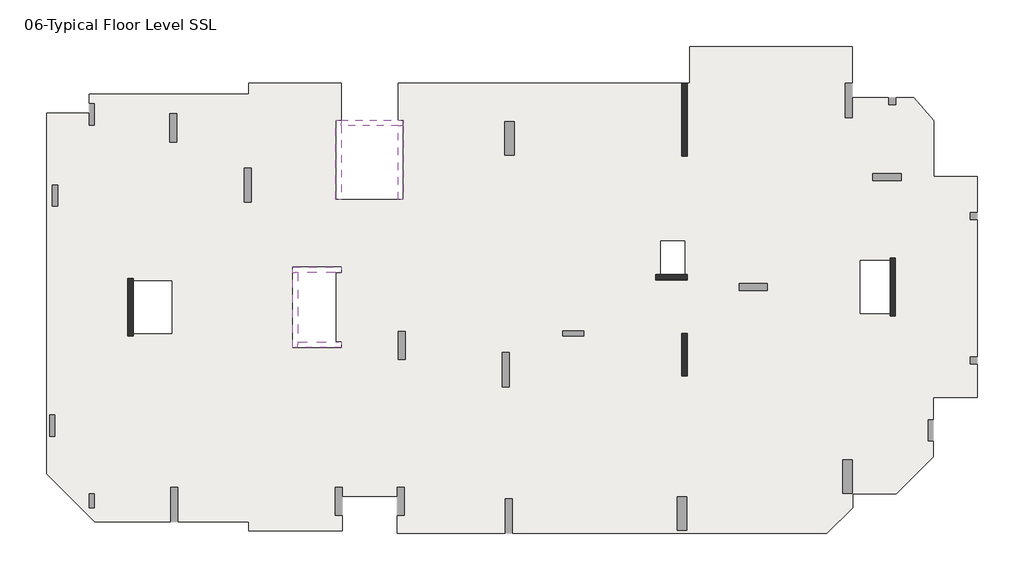
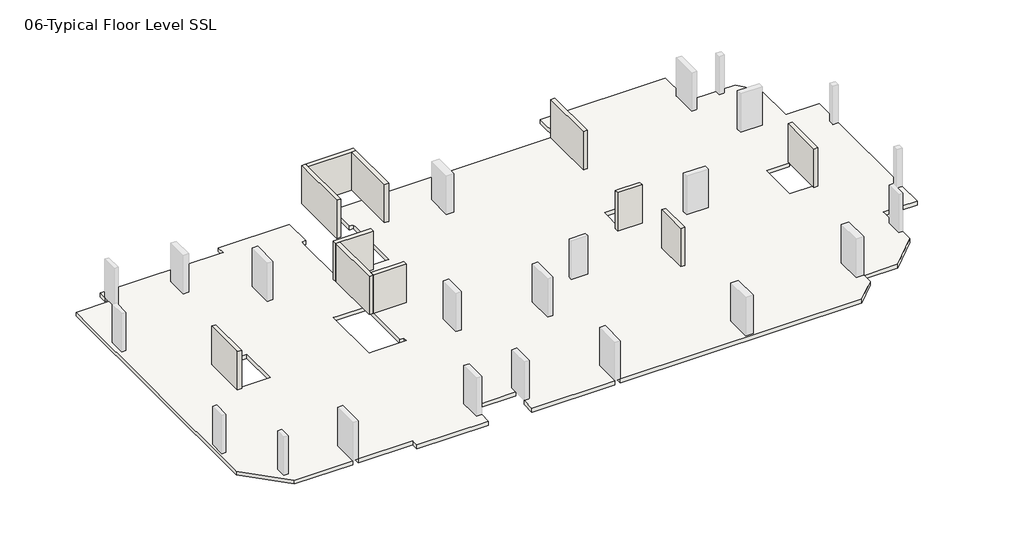
# One storey, part 1 of 2: 11 walls, 1 slab.
"""IFC4 building model written with IfcOpenShell, lengths in millimetres."""

import ifcopenshell
import ifcopenshell.guid

model = None  # the IFC model being written
_history = None  # IfcOwnerHistory: only IFC2X3 demands one
_inside = {}  # id of a spatial element -> (the spatial element, [elements in it])
_under = {}  # id of a project, library or spatial element -> (it, [spatial elements below it])
_declared = {}  # id of a project -> (the project, [libraries it declares])
_typed = {}  # id of a type object -> (the type object, [elements of that type])
_made_of = {}  # id of a material, layer set ... -> (it, [elements and type objects made of it])


def new_model(schema):
    """Start an empty IFC model of exactly this schema.

    Asked for "IFC4X3", IfcOpenShell would pick the latest addendum, in which some entities
    have other attributes; the version numbers below select the first issue.
    IFC2X3 requires an IfcOwnerHistory on every rooted entity: one is made here for all.
    """
    global model, _history
    if schema == "IFC4X3":
        model = ifcopenshell.file(schema_version=(4, 3, 0, 0))
    else:
        model = ifcopenshell.file(schema=schema)
    _inside.clear()
    _under.clear()
    _declared.clear()
    _typed.clear()
    _made_of.clear()
    _history = None
    if model.schema == "IFC2X3":
        org = make("IfcOrganization", Name="unknown")
        user = make(
            "IfcPersonAndOrganization",
            ThePerson=make("IfcPerson", FamilyName="unknown"),
            TheOrganization=org,
        )
        app = make(
            "IfcApplication",
            ApplicationDeveloper=org,
            Version="unknown",
            ApplicationFullName="unknown",
            ApplicationIdentifier="unknown",
        )
        _history = make(
            "IfcOwnerHistory",
            OwningUser=user,
            OwningApplication=app,
            ChangeAction="ADDED",
            CreationDate=0,
        )
    return model


def make(cls, **values):
    """One entity of the class cls with the attributes given. An attribute that is None is left unset."""
    return model.create_entity(
        cls, **{name: value for name, value in values.items() if value is not None}
    )


def rooted(cls, **values):
    """An entity with a GlobalId (a new one), such as an element, a storey or a relation."""
    return make(cls, GlobalId=ifcopenshell.guid.new(), OwnerHistory=_history, **values)


def si_unit(unit_type, name, prefix=None):
    """IfcSIUnit, for example si_unit("LENGTHUNIT", "METRE", prefix="MILLI")."""
    return make("IfcSIUnit", UnitType=unit_type, Prefix=prefix, Name=name)


def assignment(units):
    """IfcUnitAssignment: the units of a project."""
    return None if units is None else make("IfcUnitAssignment", Units=units)


def point(xyz):
    """IfcCartesianPoint."""
    return None if xyz is None else make("IfcCartesianPoint", Coordinates=xyz)


def direction(xyz):
    """IfcDirection."""
    return None if xyz is None else make("IfcDirection", DirectionRatios=xyz)


def frame(location, z_axis=None, x_axis=None):
    """IfcAxis2Placement3D, a coordinate frame: its origin and axes. An axis left out is left unset."""
    return make(
        "IfcAxis2Placement3D",
        Location=point(location),
        Axis=direction(z_axis),
        RefDirection=direction(x_axis),
    )


def origin():
    """The frame at (0, 0, 0) with its axes left unset."""
    return frame((0.0, 0.0, 0.0))


def place(relative_to, where):
    """IfcLocalPlacement: puts the frame where relative to a parent placement (None: the world)."""
    return make(
        "IfcLocalPlacement", PlacementRelTo=relative_to, RelativePlacement=where
    )


def context(
    kind, dimensions, precision=None, world=None, true_north=None, identifier=None
):
    """IfcGeometricRepresentationContext, for example the 3D "Model" context."""
    return make(
        "IfcGeometricRepresentationContext",
        ContextIdentifier=identifier,
        ContextType=kind,
        CoordinateSpaceDimension=dimensions,
        Precision=precision,
        WorldCoordinateSystem=world,
        TrueNorth=true_north,
    )


def project(units=None, contexts=None):
    """IfcProject with its units and contexts."""
    return rooted(
        "IfcProject",
        Name="project",
        RepresentationContexts=contexts,
        UnitsInContext=assignment(units),
    )


def spatial(cls, under=None, at=None, **own):
    """A site, building, storey or space (cls), placed at a placement, below another one or the project."""
    s = rooted(cls, ObjectPlacement=at, **own)
    if under is not None:
        _under.setdefault(under.id(), (under, []))[1].append(s)
    return s


def faces_of(points, faces, orient=None, outer=None):
    """IfcFace entities. A face is a list of loops; a loop is a list of indices into points, from 0.

    orient and outer hold one flag for each loop. By default every Orientation is true, the
    first loop of a face is its IfcFaceOuterBound and the others are IfcFaceBound.
    """
    made = []
    for i, loops in enumerate(faces):
        bounds = []
        for j, loop in enumerate(loops):
            is_outer = j == 0 if outer is None else outer[i][j]
            bounds.append(
                make(
                    "IfcFaceOuterBound" if is_outer else "IfcFaceBound",
                    Bound=make("IfcPolyLoop", Polygon=[points[k] for k in loop]),
                    Orientation=True if orient is None else orient[i][j],
                )
            )
        made.append(make("IfcFace", Bounds=bounds))
    return made


def faceted_brep(points, faces, orient=None, outer=None, voids=None):
    """IfcFacetedBrep: a solid bounded by flat faces; with voids (closed shells), ...WithVoids."""
    shared = [point(p) for p in points]
    hull = make("IfcClosedShell", CfsFaces=faces_of(shared, faces, orient, outer))
    if voids is None:
        return make("IfcFacetedBrep", Outer=hull)
    return make(
        "IfcFacetedBrepWithVoids",
        Outer=hull,
        Voids=[
            make(cls, CfsFaces=faces_of(shared, fs, o, b)) for cls, fs, o, b in voids
        ],
    )


def shape(context_of_items, identifier, shape_type, items):
    """IfcShapeRepresentation: the items that make up one representation, for example the "Body"."""
    return make(
        "IfcShapeRepresentation",
        ContextOfItems=context_of_items,
        RepresentationIdentifier=identifier,
        RepresentationType=shape_type,
        Items=items,
    )


def made_of(thing, what):
    """Note that an element or type object is made of a material, layer set ...; save() writes the relation."""
    if what is not None:
        _made_of.setdefault(what.id(), (what, []))[1].append(thing)
    return thing


def element(
    cls,
    number,
    at=None,
    inside=None,
    cuts=None,
    type_object=None,
    material=None,
    context=None,
    identifier="Body",
    shape_type=None,
    held_by="IfcProductDefinitionShape",
    body=None,
    shapes=None,
    **own,
):
    """One element of the class cls, such as IfcWall. Its Tag is "e" and its number.

    at: its placement. inside: the storey or other place that contains it. cuts: it is an
    opening in that element (IfcRelVoidsElement). A single representation is given by context,
    identifier, shape_type and body (its items); several are given by shapes. held_by: the class
    of the entity that holds the representations. save() writes the other relations.
    """
    e = rooted(cls, Tag="e%d" % number, ObjectPlacement=at, **own)
    if body is not None:
        shapes = [shape(context, identifier, shape_type, body)]
    if shapes is not None:
        e.Representation = make(held_by, Representations=shapes)
    if inside is not None:
        _inside.setdefault(inside.id(), (inside, []))[1].append(e)
    if cuts is not None:
        rooted(
            "IfcRelVoidsElement", RelatingBuildingElement=cuts, RelatedOpeningElement=e
        )
    if type_object is not None:
        _typed.setdefault(type_object.id(), (type_object, []))[1].append(e)
    return made_of(e, material)


def aggregate(whole, parts):
    """IfcRelAggregates: a whole, such as a stair, and the parts it consists of."""
    return rooted("IfcRelAggregates", RelatingObject=whole, RelatedObjects=parts)


def save(model, path):
    """Write the relations noted so far, then the file.

    IfcRelAggregates (storeys below a building ...), IfcRelContainedInSpatialStructure (elements
    in a storey), IfcRelDefinesByType, IfcRelAssociatesMaterial and IfcRelDeclares: one each for
    every whole, place, type object, material and project.
    """
    for whole, parts in _under.values():
        aggregate(whole, parts)
    for where, things in _inside.values():
        rooted(
            "IfcRelContainedInSpatialStructure",
            RelatedElements=things,
            RelatingStructure=where,
        )
    for kind, things in _typed.values():
        rooted("IfcRelDefinesByType", RelatedObjects=things, RelatingType=kind)
    for what, things in _made_of.values():
        rooted("IfcRelAssociatesMaterial", RelatedObjects=things, RelatingMaterial=what)
    for by, libraries in _declared.values():
        rooted("IfcRelDeclares", RelatingContext=by, RelatedDefinitions=libraries)
    model.write(path)


model = new_model("IFC4")

# Units and contexts
model_context = context("Model", 3, world=origin())
ifc_project = project(units=[si_unit("LENGTHUNIT", "METRE", prefix="MILLI")], contexts=[model_context])

# Site, building, storey
site = spatial("IfcSite", under=ifc_project)
building = spatial("IfcBuilding", under=site)
storey = spatial("IfcBuildingStorey", under=building, Name="06-Typical Floor Level SSL", Elevation=12000.0)

# Slab
placement = place(None, origin())
element("IfcSlab", 1, ObjectType="Generic 300mm", at=placement, inside=storey, context=model_context, shape_type="Brep", body=[
    faceted_brep([(36192.0021644, 24072.000519, 11700.0), (36192.0021644, 26172.000519, 11700.0), (45446.0007483, 26172.000519, 11700.0), (45446.0007483, 24087.0, 11700.0), (45046.0007483, 24087.0, 11700.0), (45046.0007483, 22137.0, 11700.0), (45446.0007483, 22137.0, 11700.0), (45446.0007483, 23252.0000315, 11700.0), (47498.6337868, 23252.0000315, 11700.0), (47498.6337868, 22852.0, 11700.0), (47898.6337868, 22852.0, 11700.0), (47898.6337868, 23252.0000315, 11700.0), (48936.764334, 23252.0000315, 11700.0), (50076.0016214, 21956.8283806, 11700.0), (50076.0016214, 18780.0084406, 11700.0), (52549.9999998, 18780.0084406, 11700.0), (52549.9999998, 16712.0, 11700.0), (52149.9999998, 16712.0, 11700.0), (52149.9999998, 16312.0, 11700.0), (52549.9999998, 16312.0, 11700.0), (52549.9999998, 8504.0039609, 11700.0), (52149.9999998, 8504.0039609, 11700.0), (52149.9999998, 8104.0039609, 11700.0), (52549.9999998, 8104.0039609, 11700.0), (52549.9999998, 6204.0084406, 11700.0), (50046.0009271, 6204.0084406, 11700.0), (50046.0009271, 4931.9999929, 11700.0), (49746.0009271, 4931.9999929, 11700.0), (49746.0009271, 3731.9999929, 11700.0), (50046.0009271, 3731.9999929, 11700.0), (50046.0009271, 2810.5958657, 11700.0), (47943.4055804, 708.000519, 11700.0), (45456.0017287, 708.000519, 11700.0), (45456.0017287, -61.7051085, 11700.0), (43990.7023722, -1527.004465, 11700.0), (26113.9999998, -1527.004465, 11700.0), (26113.9999998, 422.995535, 11700.0), (25713.9999998, 422.995535, 11700.0), (25713.9999998, -1527.004465, 11700.0), (19569.9997488, -1527.004465, 11700.0), (19569.9997488, -512.0044652, 11700.0), (19969.9997488, -512.0044652, 11700.0), (19969.9997488, 1087.9955348, 11700.0), (19569.9997488, 1087.9955348, 11700.0), (19569.9997488, 564.000519, 11700.0), (16429.9999981, 564.000519, 11700.0), (16429.9999981, 1088.0, 11700.0), (16029.9999981, 1088.0, 11700.0), (16029.9999981, -512.0, 11700.0), (16429.9999981, -512.0, 11700.0), (16429.9999981, -1391.999481, 11700.0), (11136.0000923, -1391.999481, 11700.0), (11136.0000923, -866.9999847, 11700.0), (7082.0000416, -866.9999847, 11700.0), (7082.0000416, 1083.0000153, 11700.0), (6682.0000416, 1083.0000153, 11700.0), (6682.0000416, -866.9999847, 11700.0), (2364.4419097, -866.9999847, 11700.0), (-372.0, 1869.441925, 11700.0), (-372.0, 22380.0004589, 11700.0), (2052.0, 22380.0004589, 11700.0), (2052.0, 21708.0000656, 11700.0), (2352.0, 21708.0000656, 11700.0), (2352.0, 22908.0000656, 11700.0), (2052.0, 22908.0000656, 11700.0), (2052.0, 23472.000519, 11700.0), (11136.0000923, 23472.000519, 11700.0), (11136.0000923, 24072.000519, 11700.0), (16380.0000168, 24072.000519, 11700.0), (16380.0000168, 21972.0, 11700.0), (16079.9999997, 21972.0, 11700.0), (16079.9999997, 21672.0, 11700.0), (16079.9999997, 17468.0, 11700.0), (16379.9999997, 17468.0, 11700.0), (19619.9999997, 17468.0, 11700.0), (19919.9999997, 17468.0, 11700.0), (19919.9999997, 21672.0, 11700.0), (19919.9999997, 21972.0, 11700.0), (19619.9997365, 21972.0, 11700.0), (19619.9997365, 24072.000519, 11700.0), (35747.9999998, 24072.000519, 11700.0), (35747.9999998, 19932.0, 11700.0), (36047.9999998, 19932.0, 11700.0), (36047.9999998, 24072.000519, 11700.0), (16079.9999907, 9359.999998, 11700.0), (16079.9999907, 13320.0000002, 11700.0), (16380.0000168, 13320.0000002, 11700.0), (16380.0000168, 13620.0000002, 11700.0), (13919.9999907, 13620.0000002, 11700.0), (13619.9999907, 13620.0000002, 11700.0), (13619.9999907, 13320.0000002, 11700.0), (13619.9999907, 9359.999998, 11700.0), (13619.9999907, 9059.999998, 11700.0), (13919.9999907, 9059.999998, 11700.0), (16380.0000168, 9059.999998, 11700.0), (16380.0000168, 9359.999998, 11700.0), (257.9999999, 17088.0, 11700.0), (257.9999999, 18288.0, 11700.0), (-42.0000001, 18288.0, 11700.0), (-42.0000001, 17088.0, 11700.0), (108.001803, 4001.9999858, 11700.0), (108.001803, 5201.9999858, 11700.0), (-191.998197, 5201.9999858, 11700.0), (-191.998197, 4001.9999858, 11700.0), (30175.9999998, 9996.0000019, 11700.0), (28975.9999998, 9996.0000019, 11700.0), (28975.9999998, 9696.0000019, 11700.0), (30175.9999998, 9696.0000019, 11700.0), (7021.9999999, 20740.0000078, 11700.0), (7021.9999999, 22340.0000078, 11700.0), (6621.9999999, 22340.0000078, 11700.0), (6621.9999999, 20740.0000078, 11700.0), (48205.9993605, 18950.0, 11700.0), (46605.9993605, 18950.0, 11700.0), (46605.9993605, 18550.0, 11700.0), (48205.9993605, 18550.0, 11700.0), (20030.000009, 8355.9999979, 11700.0), (20030.000009, 9955.9999979, 11700.0), (19630.000009, 9955.9999979, 11700.0), (19630.000009, 8355.9999979, 11700.0), (11270.0000427, 17312.9999996, 11700.0), (11270.0000427, 19262.9999996, 11700.0), (10870.0000427, 19262.9999996, 11700.0), (10870.0000427, 17312.9999996, 11700.0), (40598.0014887, 12692.0079212, 11700.0), (38998.0014887, 12692.0079212, 11700.0), (38998.0014887, 12292.0079212, 11700.0), (40598.0014887, 12292.0079212, 11700.0), (2352.0, -72.0, 11700.0), (2352.0, 728.0, 11700.0), (2052.0, 728.0, 11700.0), (2052.0, -72.0, 11700.0), (25934.0000455, 6801.0001824, 11700.0), (25934.0000455, 8751.0001824, 11700.0), (25534.0000455, 8751.0001824, 11700.0), (25534.0000455, 6801.0001824, 11700.0), (36035.9999998, -1351.9992017, 11700.0), (36035.9999998, 548.0007983, 11700.0), (35485.9999998, 548.0007983, 11700.0), (35485.9999998, -1351.9992017, 11700.0), (45443.9999998, 748.0, 11700.0), (45443.9999998, 2648.0, 11700.0), (44893.9999998, 2648.0, 11700.0), (44893.9999998, 748.0, 11700.0), (26218.9999998, 20000.0, 11700.0), (26218.9999998, 21900.0, 11700.0), (25668.9999998, 21900.0, 11700.0), (25668.9999998, 20000.0, 11700.0), (4248.0000025, 12984.0000001, 11700.0), (4248.0000025, 9696.0, 11700.0), (4548.0000025, 9696.0, 11700.0), (4548.0000025, 9840.0000003, 11700.0), (6743.9999995, 9840.0000003, 11700.0), (6743.9999995, 12840.0000003, 11700.0), (4548.0000034, 12840.0000003, 11700.0), (4548.0000025, 12984.0000001, 11700.0), (34248.0015201, 12899.9999992, 11700.0), (36048.0015201, 12899.9999992, 11700.0), (36048.0015201, 13199.9999992, 11700.0), (35904.002157, 13199.9999992, 11700.0), (35904.002157, 15108.0000083, 11700.0), (34548.0015145, 15108.0000083, 11700.0), (34548.0015145, 13199.9999992, 11700.0), (34248.0015201, 13199.9999992, 11700.0), (35748.0054035, 9840.0000002, 11700.0), (35748.0054035, 7428.0000762, 11700.0), (36048.0054035, 7428.0000762, 11700.0), (36048.0054035, 9840.0000002, 11700.0), (47580.0014811, 14136.0000002, 11700.0), (47580.0014811, 13992.0079177, 11700.0), (45900.001729, 13992.0079177, 11700.0), (45900.001729, 10992.0079181, 11700.0), (47580.0014798, 10992.0079181, 11700.0), (47580.0014811, 10848.0079202, 11700.0), (47880.0014811, 10848.0079202, 11700.0), (47880.0014811, 14136.0000002, 11700.0), (36192.0021644, 26172.000519, 12000.0), (36192.0021644, 24072.000519, 12000.0), (36047.9999998, 24072.000519, 12000.0), (36047.9999998, 19932.0, 12000.0), (35747.9999998, 19932.0, 12000.0), (35747.9999998, 24072.000519, 12000.0), (19619.9997365, 24072.000519, 12000.0), (19619.9997365, 21972.0, 12000.0), (19919.9999997, 21972.0, 12000.0), (19919.9999997, 21672.0, 12000.0), (19919.9999997, 17468.0, 12000.0), (19619.9999997, 17468.0, 12000.0), (16379.9999997, 17468.0, 12000.0), (16079.9999997, 17468.0, 12000.0), (16079.9999997, 21672.0, 12000.0), (16079.9999997, 21972.0, 12000.0), (16380.0000168, 21972.0, 12000.0), (16380.0000168, 24072.000519, 12000.0), (11136.0000923, 24072.000519, 12000.0), (11136.0000923, 23472.000519, 12000.0), (2052.0, 23472.000519, 12000.0), (2052.0, 22908.0000656, 12000.0), (2352.0, 22908.0000656, 12000.0), (2352.0, 21708.0000656, 12000.0), (2052.0, 21708.0000656, 12000.0), (2052.0, 22380.0004589, 12000.0), (-372.0, 22380.0004589, 12000.0), (-372.0, 1869.441925, 12000.0), (2364.4419097, -866.9999847, 12000.0), (6682.0000416, -866.9999847, 12000.0), (6682.0000416, 1083.0000153, 12000.0), (7082.0000416, 1083.0000153, 12000.0), (7082.0000416, -866.9999847, 12000.0), (11136.0000923, -866.9999847, 12000.0), (11136.0000923, -1391.999481, 12000.0), (16429.9999981, -1391.999481, 12000.0), (16429.9999981, -512.0, 12000.0), (16029.9999981, -512.0, 12000.0), (16029.9999981, 1088.0, 12000.0), (16429.9999981, 1088.0, 12000.0), (16429.9999981, 564.000519, 12000.0), (19569.9997488, 564.000519, 12000.0), (19569.9997488, 1087.9955348, 12000.0), (19969.9997488, 1087.9955348, 12000.0), (19969.9997488, -512.0044652, 12000.0), (19569.9997488, -512.0044652, 12000.0), (19569.9997488, -1527.004465, 12000.0), (25713.9999998, -1527.004465, 12000.0), (25713.9999998, 422.995535, 12000.0), (26113.9999998, 422.995535, 12000.0), (26113.9999998, -1527.004465, 12000.0), (43990.7023722, -1527.004465, 12000.0), (45456.0017287, -61.7051085, 12000.0), (45456.0017287, 708.000519, 12000.0), (47943.4055804, 708.000519, 12000.0), (50046.0009271, 2810.5958657, 12000.0), (50046.0009271, 3731.9999929, 12000.0), (49746.0009271, 3731.9999929, 12000.0), (49746.0009271, 4931.9999929, 12000.0), (50046.0009271, 4931.9999929, 12000.0), (50046.0009271, 6204.0084406, 12000.0), (52549.9999998, 6204.0084406, 12000.0), (52549.9999998, 8104.0039609, 12000.0), (52149.9999998, 8104.0039609, 12000.0), (52149.9999998, 8504.0039609, 12000.0), (52549.9999998, 8504.0039609, 12000.0), (52549.9999998, 16312.0, 12000.0), (52149.9999998, 16312.0, 12000.0), (52149.9999998, 16712.0, 12000.0), (52549.9999998, 16712.0, 12000.0), (52549.9999998, 18780.0084406, 12000.0), (50076.0016214, 18780.0084406, 12000.0), (50076.0016214, 21956.8283806, 12000.0), (48936.764334, 23252.0000315, 12000.0), (47898.6337868, 23252.0000315, 12000.0), (47898.6337868, 22852.0, 12000.0), (47498.6337868, 22852.0, 12000.0), (47498.6337868, 23252.0000315, 12000.0), (45446.0006898, 23252.0000315, 12000.0), (45446.0007483, 22137.0, 12000.0), (45046.0007483, 22137.0, 12000.0), (45046.0007483, 24087.0, 12000.0), (45446.0007483, 24087.0, 12000.0), (45446.0007483, 26172.000519, 12000.0), (16079.9999907, 13320.0000002, 12000.0), (16079.9999907, 9359.999998, 12000.0), (16380.0000168, 9359.999998, 12000.0), (16380.0000168, 9059.999998, 12000.0), (13919.9999907, 9059.999998, 12000.0), (13619.9999907, 9059.999998, 12000.0), (13619.9999907, 9359.999998, 12000.0), (13619.9999907, 13320.0000002, 12000.0), (13619.9999907, 13620.0000002, 12000.0), (13919.9999907, 13620.0000002, 12000.0), (16380.0000168, 13620.0000002, 12000.0), (16380.0000168, 13320.0000002, 12000.0), (257.9999999, 18288.0, 12000.0), (257.9999999, 17088.0, 12000.0), (-42.0000001, 17088.0, 12000.0), (-42.0000001, 18288.0, 12000.0), (108.001803, 5201.9999858, 12000.0), (108.001803, 4001.9999858, 12000.0), (-191.998197, 4001.9999858, 12000.0), (-191.998197, 5201.9999858, 12000.0), (28975.9999998, 9996.0000019, 12000.0), (30175.9999998, 9996.0000019, 12000.0), (30175.9999998, 9696.0000019, 12000.0), (28975.9999998, 9696.0000019, 12000.0), (7021.9999999, 22340.0000078, 12000.0), (7021.9999999, 20740.0000078, 12000.0), (6621.9999999, 20740.0000078, 12000.0), (6621.9999999, 22340.0000078, 12000.0), (46605.9993605, 18950.0, 12000.0), (48205.9993605, 18950.0, 12000.0), (48205.9993605, 18550.0, 12000.0), (46605.9993605, 18550.0, 12000.0), (20030.000009, 9955.9999979, 12000.0), (20030.000009, 8355.9999979, 12000.0), (19630.000009, 8355.9999979, 12000.0), (19630.000009, 9955.9999979, 12000.0), (11270.0000427, 19262.9999996, 12000.0), (11270.0000427, 17312.9999996, 12000.0), (10870.0000427, 17312.9999996, 12000.0), (10870.0000427, 19262.9999996, 12000.0), (38998.0014887, 12692.0079212, 12000.0), (40598.0014887, 12692.0079212, 12000.0), (40598.0014887, 12292.0079212, 12000.0), (38998.0014887, 12292.0079212, 12000.0), (2352.0, 728.0, 12000.0), (2352.0, -72.0, 12000.0), (2052.0, -72.0, 12000.0), (2052.0, 728.0, 12000.0), (25934.0000455, 8751.0001824, 12000.0), (25934.0000455, 6801.0001824, 12000.0), (25534.0000455, 6801.0001824, 12000.0), (25534.0000455, 8751.0001824, 12000.0), (36035.9999998, 548.0007983, 12000.0), (36035.9999998, -1351.9992017, 12000.0), (35485.9999998, -1351.9992017, 12000.0), (35485.9999998, 548.0007983, 12000.0), (45443.9999998, 2648.0, 12000.0), (45443.9999998, 748.0, 12000.0), (44893.9999998, 748.0, 12000.0), (44893.9999998, 2648.0, 12000.0), (26218.9999998, 21900.0, 12000.0), (26218.9999998, 20000.0, 12000.0), (25668.9999998, 20000.0, 12000.0), (25668.9999998, 21900.0, 12000.0), (4248.0000025, 9696.0, 12000.0), (4248.0000025, 12984.0000001, 12000.0), (4548.0000025, 12984.0000001, 12000.0), (4548.0000025, 12840.0000003, 12000.0), (6743.9999995, 12840.0000003, 12000.0), (6743.9999995, 9840.0000003, 12000.0), (4548.0000034, 9840.0000003, 12000.0), (4548.0000025, 9696.0, 12000.0), (36048.0015201, 12899.9999992, 12000.0), (34248.0015201, 12899.9999992, 12000.0), (34248.0015201, 13199.9999992, 12000.0), (34548.0015145, 13199.9999992, 12000.0), (34548.0015145, 15108.0000083, 12000.0), (35904.002157, 15108.0000083, 12000.0), (35904.002157, 13199.9999992, 12000.0), (36048.0015201, 13199.9999992, 12000.0), (35748.0054035, 7428.0000762, 12000.0), (35748.0054035, 9840.0000002, 12000.0), (36048.0054035, 9840.0000002, 12000.0), (36048.0054035, 7428.0000762, 12000.0), (47880.0014811, 14136.0000002, 12000.0), (47880.0014811, 10848.0079202, 12000.0), (47580.0014811, 10848.0079202, 12000.0), (47580.0014811, 10992.0079181, 12000.0), (45900.001729, 10992.0079181, 12000.0), (45900.001729, 13992.0079177, 12000.0), (47580.0014798, 13992.0079177, 12000.0), (47580.0014811, 14136.0000002, 12000.0)], [[[0, 1, 2, 3, 4, 5, 6, 7, 8, 9, 10, 11, 12, 13, 14, 15, 16, 17, 18, 19, 20, 21, 22, 23, 24, 25, 26, 27, 28, 29, 30, 31, 32, 33, 34, 35, 36, 37, 38, 39, 40, 41, 42, 43, 44, 45, 46, 47, 48, 49, 50, 51, 52, 53, 54, 55, 56, 57, 58, 59, 60, 61, 62, 63, 64, 65, 66, 67, 68, 69, 70, 71, 72, 73, 74, 75, 76, 77, 78, 79, 80, 81, 82, 83], [84, 85, 86, 87, 88, 89, 90, 91, 92, 93, 94, 95], [96, 97, 98, 99], [100, 101, 102, 103], [104, 105, 106, 107], [108, 109, 110, 111], [112, 113, 114, 115], [116, 117, 118, 119], [120, 121, 122, 123], [124, 125, 126, 127], [128, 129, 130, 131], [132, 133, 134, 135], [136, 137, 138, 139], [140, 141, 142, 143], [144, 145, 146, 147], [148, 149, 150, 151, 152, 153, 154, 155], [156, 157, 158, 159, 160, 161, 162, 163], [164, 165, 166, 167], [168, 169, 170, 171, 172, 173, 174, 175]], [[176, 177, 178, 179, 180, 181, 182, 183, 184, 185, 186, 187, 188, 189, 190, 191, 192, 193, 194, 195, 196, 197, 198, 199, 200, 201, 202, 203, 204, 205, 206, 207, 208, 209, 210, 211, 212, 213, 214, 215, 216, 217, 218, 219, 220, 221, 222, 223, 224, 225, 226, 227, 228, 229, 230, 231, 232, 233, 234, 235, 236, 237, 238, 239, 240, 241, 242, 243, 244, 245, 246, 247, 248, 249, 250, 251, 252, 253, 254, 255, 256, 257, 258, 259], [260, 261, 262, 263, 264, 265, 266, 267, 268, 269, 270, 271], [272, 273, 274, 275], [276, 277, 278, 279], [280, 281, 282, 283], [284, 285, 286, 287], [288, 289, 290, 291], [292, 293, 294, 295], [296, 297, 298, 299], [300, 301, 302, 303], [304, 305, 306, 307], [308, 309, 310, 311], [312, 313, 314, 315], [316, 317, 318, 319], [320, 321, 322, 323], [324, 325, 326, 327, 328, 329, 330, 331], [332, 333, 334, 335, 336, 337, 338, 339], [340, 341, 342, 343], [344, 345, 346, 347, 348, 349, 350, 351]], [[68, 193, 192, 69]], [[182, 79, 78, 183]], [[79, 182, 181, 80]], [[177, 0, 83, 178]], [[1, 0, 177, 176]], [[2, 1, 176, 259]], [[3, 2, 259, 258]], [[249, 12, 11, 250]], [[7, 254, 253, 8]], [[13, 12, 249, 248]], [[14, 13, 248, 247]], [[15, 14, 247, 246]], [[15, 246, 245, 16]], [[237, 24, 23, 238]], [[19, 242, 241, 20]], [[25, 24, 237, 236]], [[25, 236, 235, 26]], [[30, 29, 232, 231]], [[32, 31, 230, 229]], [[33, 32, 229, 228]], [[34, 33, 228, 227]], [[34, 227, 226, 35]], [[222, 39, 38, 223]], [[39, 222, 221, 40]], [[45, 44, 217, 216]], [[211, 50, 49, 212]], [[51, 50, 211, 210]], [[52, 51, 210, 209]], [[52, 209, 208, 53]], [[204, 57, 56, 205]], [[58, 57, 204, 203]], [[59, 58, 203, 202]], [[60, 59, 202, 201]], [[196, 65, 64, 197]], [[66, 65, 196, 195]], [[67, 66, 195, 194]], [[68, 67, 194, 193]], [[85, 84, 261, 260]], [[62, 199, 198, 63]], [[199, 62, 61, 200]], [[200, 61, 60, 201]], [[63, 198, 197, 64]], [[96, 273, 272, 97]], [[273, 96, 99, 274]], [[274, 99, 98, 275]], [[275, 98, 97, 272]], [[100, 277, 276, 101]], [[277, 100, 103, 278]], [[278, 103, 102, 279]], [[279, 102, 101, 276]], [[28, 233, 232, 29]], [[233, 28, 27, 234]], [[234, 27, 26, 235]], [[104, 281, 280, 105]], [[281, 104, 107, 282]], [[282, 107, 106, 283]], [[283, 106, 105, 280]], [[108, 285, 284, 109]], [[285, 108, 111, 286]], [[286, 111, 110, 287]], [[287, 110, 109, 284]], [[41, 220, 219, 42]], [[220, 41, 40, 221]], [[43, 218, 217, 44]], [[218, 43, 42, 219]], [[112, 289, 288, 113]], [[289, 112, 115, 290]], [[290, 115, 114, 291]], [[291, 114, 113, 288]], [[116, 293, 292, 117]], [[293, 116, 119, 294]], [[294, 119, 118, 295]], [[295, 118, 117, 292]], [[215, 46, 45, 216]], [[48, 213, 212, 49]], [[213, 48, 47, 214]], [[214, 47, 46, 215]], [[120, 297, 296, 121]], [[297, 120, 123, 298]], [[298, 123, 122, 299]], [[299, 122, 121, 296]], [[207, 54, 53, 208]], [[55, 206, 205, 56]], [[206, 55, 54, 207]], [[225, 36, 35, 226]], [[37, 224, 223, 38]], [[224, 37, 36, 225]], [[6, 255, 254, 7]], [[255, 6, 5, 256]], [[256, 5, 4, 257]], [[257, 4, 3, 258]], [[124, 301, 300, 125]], [[301, 124, 127, 302]], [[302, 127, 126, 303]], [[303, 126, 125, 300]], [[128, 305, 304, 129]], [[305, 128, 131, 306]], [[306, 131, 130, 307]], [[307, 130, 129, 304]], [[132, 309, 308, 133]], [[309, 132, 135, 310]], [[310, 135, 134, 311]], [[311, 134, 133, 308]], [[136, 313, 312, 137]], [[313, 136, 139, 314]], [[314, 139, 138, 315]], [[315, 138, 137, 312]], [[140, 317, 316, 141]], [[317, 140, 143, 318]], [[318, 143, 142, 319]], [[319, 142, 141, 316]], [[144, 321, 320, 145]], [[321, 144, 147, 322]], [[322, 147, 146, 323]], [[323, 146, 145, 320]], [[70, 191, 190, 189, 72, 71]], [[191, 70, 69, 192]], [[77, 184, 183, 78]], [[184, 77, 76, 75, 186, 185]], [[271, 86, 85, 260]], [[87, 270, 269, 268, 89, 88]], [[86, 271, 270, 87]], [[89, 268, 267, 266, 265, 92, 91, 90]], [[92, 265, 264, 263, 94, 93]], [[95, 262, 261, 84]], [[262, 95, 94, 263]], [[326, 155, 154, 327]], [[150, 331, 330, 151]], [[148, 325, 324, 149]], [[155, 326, 325, 148]], [[331, 150, 149, 324]], [[156, 333, 332, 157]], [[158, 339, 338, 159]], [[334, 163, 162, 335]], [[157, 332, 339, 158]], [[333, 156, 163, 334]], [[164, 341, 340, 165]], [[166, 343, 342, 167]], [[165, 340, 343, 166]], [[341, 164, 167, 342]], [[346, 173, 172, 347]], [[168, 351, 350, 169]], [[174, 345, 344, 175]], [[173, 346, 345, 174]], [[351, 168, 175, 344]], [[82, 179, 178, 83]], [[180, 81, 80, 181]], [[179, 82, 81, 180]], [[72, 189, 188, 187, 186, 75, 74, 73]], [[329, 152, 151, 330]], [[152, 329, 328, 153]], [[153, 328, 327, 154]], [[349, 170, 169, 350]], [[170, 349, 348, 171]], [[171, 348, 347, 172]], [[160, 337, 336, 161]], [[161, 336, 335, 162]], [[337, 160, 159, 338]], [[31, 30, 231, 230]], [[18, 243, 242, 19]], [[243, 18, 17, 244]], [[244, 17, 16, 245]], [[10, 251, 250, 11]], [[251, 10, 9, 252]], [[252, 9, 8, 253]], [[22, 239, 238, 23]], [[239, 22, 21, 240]], [[240, 21, 20, 241]]]),
])

# Walls
element("IfcWall", 2, ObjectType="Shear Walls 300mm", at=placement, inside=storey, context=model_context, shape_type="Brep", body=[
    faceted_brep([(4548.0000025, 9696.0, 12000.0), (4548.0000025, 12984.0000001, 12000.0), (4548.0000025, 12984.0000001, 14700.0), (4548.0000025, 12984.0000001, 15000.0), (4548.0000025, 12840.0000003, 15000.0), (4548.0000025, 9840.0000003, 15000.0), (4548.0000025, 9696.0, 15000.0), (4548.0000025, 9696.0, 14700.0), (4248.0000025, 9696.0, 12000.0), (4248.0000025, 9696.0, 14700.0), (4248.0000025, 9696.0, 15000.0), (4248.0000025, 12984.0000001, 15000.0), (4248.0000025, 12984.0000001, 14700.0), (4248.0000025, 12984.0000001, 12000.0)], [[[0, 1, 2, 3, 4, 5, 6, 7]], [[8, 9, 10, 11, 12, 13]], [[1, 0, 8, 13]], [[3, 2, 1, 13, 12, 11]], [[6, 5, 4, 3, 11, 10]], [[0, 7, 6, 10, 9, 8]]]),
])
element("IfcWall", 3, ObjectType="Shear Walls 300mm", at=placement, inside=storey, context=model_context, shape_type="Brep", body=[
    faceted_brep([(34248.0015201, 12899.9999992, 12000.0), (36048.0015201, 12899.9999992, 12000.0), (36048.0015201, 12899.9999992, 14700.0), (36048.0015201, 12899.9999992, 15000.0), (34248.0015201, 12899.9999992, 15000.0), (34248.0015201, 12899.9999992, 14700.0), (34248.0015201, 13199.9999992, 12000.0), (34248.0015201, 13199.9999992, 14700.0), (34248.0015201, 13199.9999992, 15000.0), (34548.0015145, 13199.9999992, 15000.0), (35904.002157, 13199.9999992, 15000.0), (36048.0015201, 13199.9999992, 15000.0), (36048.0015201, 13199.9999992, 14700.0), (36048.0015201, 13199.9999992, 12000.0)], [[[0, 1, 2, 3, 4, 5]], [[6, 7, 8, 9, 10, 11, 12, 13]], [[1, 0, 6, 13]], [[3, 2, 1, 13, 12, 11]], [[4, 3, 11, 10, 9, 8]], [[0, 5, 4, 8, 7, 6]]]),
])
element("IfcWall", 4, ObjectType="Shear Walls 300mm", at=placement, inside=storey, context=model_context, shape_type="Brep", body=[
    faceted_brep([(35748.0054035, 9840.0000002, 12000.0), (35748.0054035, 7428.0000762, 12000.0), (35748.0054035, 7428.0000762, 14700.0), (35748.0054035, 7428.0000762, 15000.0), (35748.0054035, 9840.0000002, 15000.0), (35748.0054035, 9840.0000002, 14700.0), (36048.0054035, 9840.0000002, 12000.0), (36048.0054035, 9840.0000002, 14700.0), (36048.0054035, 9840.0000002, 15000.0), (36048.0054035, 7428.0000762, 15000.0), (36048.0054035, 7428.0000762, 14700.0), (36048.0054035, 7428.0000762, 12000.0)], [[[0, 1, 2, 3, 4, 5]], [[6, 7, 8, 9, 10, 11]], [[1, 0, 6, 11]], [[3, 2, 1, 11, 10, 9]], [[4, 3, 9, 8]], [[0, 5, 4, 8, 7, 6]]]),
])
element("IfcWall", 5, ObjectType="Shear Walls 300mm", at=placement, inside=storey, context=model_context, shape_type="Brep", body=[
    faceted_brep([(47580.0014811, 14136.0000002, 12000.0), (47580.0014811, 10848.0079202, 12000.0), (47580.0014811, 10848.0079202, 14700.0), (47580.0014811, 10848.0079202, 15000.0), (47580.0014811, 10992.0079181, 15000.0), (47580.0014811, 13992.0079177, 15000.0), (47580.0014811, 14136.0000002, 15000.0), (47580.0014811, 14136.0000002, 14700.0), (47880.0014811, 14136.0000002, 12000.0), (47880.0014811, 14136.0000002, 14700.0), (47880.0014811, 14136.0000002, 15000.0), (47880.0014811, 10848.0079202, 15000.0), (47880.0014811, 10848.0079202, 14700.0), (47880.0014811, 10848.0079202, 12000.0)], [[[0, 1, 2, 3, 4, 5, 6, 7]], [[8, 9, 10, 11, 12, 13]], [[1, 0, 8, 13]], [[3, 2, 1, 13, 12, 11]], [[6, 5, 4, 3, 11, 10]], [[0, 7, 6, 10, 9, 8]]]),
])
element("IfcWall", 6, ObjectType="Shear Walls 300mm", at=placement, inside=storey, context=model_context, shape_type="Brep", body=[
    faceted_brep([(36047.9999998, 19932.0, 12000.0), (36047.9999998, 24072.0078999, 12000.0), (36047.9999998, 24072.0078999, 15000.0), (36047.9999998, 19932.0, 15000.0), (36047.9999998, 19932.0, 14700.0), (35747.9999998, 19932.0, 12000.0), (35747.9999998, 19932.0, 14700.0), (35747.9999998, 19932.0, 15000.0), (35747.9999998, 24072.0078999, 15000.0), (35747.9999998, 24072.0078999, 12000.0)], [[[0, 1, 2, 3, 4]], [[5, 6, 7, 8, 9]], [[1, 0, 5, 9]], [[2, 1, 9, 8]], [[3, 2, 8, 7]], [[0, 4, 3, 7, 6, 5]]]),
])
element("IfcWall", 7, ObjectType="Shear Walls 300mm", at=placement, inside=storey, context=model_context, shape_type="Brep", body=[
    faceted_brep([(16379.9999997, 21972.0, 18000.0), (16379.9999997, 21672.0, 18000.0), (16379.9999997, 17468.0, 18000.0), (16379.9999997, 17468.0, 15000.0), (16379.9999997, 21672.0, 15000.0), (16379.9999997, 21972.0, 15000.0), (16079.9999997, 17468.0, 18000.0), (16079.9999997, 21972.0, 18000.0), (16079.9999997, 21972.0, 17700.0), (16079.9999997, 21972.0, 15000.0), (16079.9999997, 17468.0, 15000.0), (16079.9999997, 17468.0, 17700.0)], [[[0, 1, 2, 3, 4, 5]], [[6, 7, 8, 9, 10, 11]], [[2, 1, 0, 7, 6]], [[2, 6, 11, 10, 3]], [[3, 10, 9, 5, 4]], [[0, 5, 9, 8, 7]]]),
])
element("IfcWall", 8, ObjectType="Shear Walls 300mm", at=placement, inside=storey, context=model_context, shape_type="Brep", body=[
    faceted_brep([(16379.9999997, 21972.0, 18000.0), (19619.9997365, 21972.0, 18000.0), (19919.9999997, 21972.0, 18000.0), (19919.9999997, 21972.0, 17700.0), (19919.9999997, 21972.0, 15000.0), (16379.9999997, 21972.0, 15000.0), (19919.9999997, 21672.0, 18000.0), (19619.9999997, 21672.0, 18000.0), (16379.9999997, 21672.0, 18000.0), (16379.9999997, 21672.0, 15000.0), (19619.9999997, 21672.0, 15000.0), (19919.9999997, 21672.0, 15000.0)], [[[0, 1, 2, 3, 4, 5]], [[6, 7, 8, 9, 10, 11]], [[2, 1, 0, 8, 7, 6]], [[8, 0, 5, 9]], [[9, 5, 4, 11, 10]], [[4, 3, 2, 6, 11]]]),
])
element("IfcWall", 9, ObjectType="Shear Walls 300mm", at=placement, inside=storey, context=model_context, shape_type="Brep", body=[
    faceted_brep([(19919.9999997, 21672.0, 18000.0), (19919.9999997, 17468.0, 18000.0), (19919.9999997, 17468.0, 17700.0), (19919.9999997, 17468.0, 15000.0), (19919.9999997, 21672.0, 15000.0), (19619.9999997, 17468.0, 18000.0), (19619.9999997, 21672.0, 18000.0), (19619.9999997, 21672.0, 15000.0), (19619.9999997, 17468.0, 15000.0)], [[[0, 1, 2, 3, 4]], [[5, 6, 7, 8]], [[1, 0, 6, 5]], [[1, 5, 8, 3, 2]], [[6, 0, 4, 7]], [[4, 3, 8, 7]]]),
])
element("IfcWall", 10, ObjectType="Shear Walls 300mm", at=placement, inside=storey, context=model_context, shape_type="Brep", body=[
    faceted_brep([(16380.0000168, 13320.0000002, 18000.0), (16079.9999907, 13320.0000002, 18000.0), (13919.9999907, 13320.0000002, 18000.0), (13619.9999907, 13320.0000002, 18000.0), (13619.9999907, 13320.0000002, 15000.0), (13919.9999907, 13320.0000002, 15000.0), (16380.0000168, 13320.0000002, 15000.0), (16380.0000168, 13320.0000002, 17700.0), (13619.9999907, 13620.0000002, 18000.0), (16380.0000168, 13620.0000002, 18000.0), (16380.0000168, 13620.0000002, 17700.0), (16380.0000168, 13620.0000002, 15000.0), (13619.9999907, 13620.0000002, 15000.0), (13619.9999907, 13620.0000002, 17700.0)], [[[0, 1, 2, 3, 4, 5, 6, 7]], [[8, 9, 10, 11, 12, 13]], [[9, 0, 7, 6, 11, 10]], [[3, 2, 1, 0, 9, 8]], [[11, 6, 5, 4, 12]], [[4, 3, 8, 13, 12]]]),
])
element("IfcWall", 11, ObjectType="Shear Walls 300mm", at=placement, inside=storey, context=model_context, shape_type="Brep", body=[
    faceted_brep([(13919.9999907, 13320.0000002, 18000.0), (13919.9999907, 9359.999998, 18000.0), (13919.9999907, 9059.999998, 18000.0), (13919.9999907, 9059.999998, 15000.0), (13919.9999907, 9359.999998, 15000.0), (13919.9999907, 13320.0000002, 15000.0), (13619.9999907, 9059.999998, 18000.0), (13619.9999907, 13320.0000002, 18000.0), (13619.9999907, 13320.0000002, 15000.0), (13619.9999907, 9059.999998, 15000.0), (13619.9999907, 9059.999998, 17700.0)], [[[0, 1, 2, 3, 4, 5]], [[6, 7, 8, 9, 10]], [[2, 1, 0, 7, 6]], [[7, 0, 5, 8]], [[8, 5, 4, 3, 9]], [[3, 2, 6, 10, 9]]]),
])
element("IfcWall", 12, ObjectType="Shear Walls 300mm", at=placement, inside=storey, context=model_context, shape_type="Brep", body=[
    faceted_brep([(13919.9999907, 9359.999998, 18000.0), (16079.9999907, 9359.999998, 18000.0), (16380.0000168, 9359.999998, 18000.0), (16380.0000168, 9359.999998, 17700.0), (16380.0000168, 9359.999998, 15000.0), (13919.9999907, 9359.999998, 15000.0), (16380.0000168, 9059.999998, 18000.0), (13919.9999907, 9059.999998, 18000.0), (13919.9999907, 9059.999998, 15000.0), (16380.0000168, 9059.999998, 15000.0), (16380.0000168, 9059.999998, 17700.0)], [[[0, 1, 2, 3, 4, 5]], [[6, 7, 8, 9, 10]], [[2, 1, 0, 7, 6]], [[2, 6, 10, 9, 4, 3]], [[7, 0, 5, 8]], [[5, 4, 9, 8]]]),
])

save(model, "model.ifc")

# Revit data of these elements
# Type "Generic 300mm"
#   Function = 0
#   Layers, outside or top first: 300 mm "Concrete-RC" (function 1)
# Type "Shear Walls 300mm"
#   Layers, outside or top first: 300 mm "Concrete-RC" (function 1)
# Element 1 (IfcSlab, "Generic 300mm")
#   Height Offset From Level = 0 mm
#   built-in parameter 1001954 = 1
#   Phase Created = New Construction
#   Materials on its faces: "Concrete-RC"
# Elements 2, 3, 4, 5, 6 (IfcWall, "Shear Walls 300mm")
#   Top Offset = 0 mm
#   Base Offset = 0 mm
#   wall height = 3000 mm
#   Phase Created = New Construction
#   Base Constraint = 06-Typical Floor Level SSL
#   Top Constraint = 07-Typical Floor Level SSL
#   Materials on its faces: "Concrete-RC"
# Elements 7, 8, 9, 10, 11, 12 (IfcWall, "Shear Walls 300mm")
#   Top Offset = 0 mm
#   Base Offset = 0 mm
#   wall height = 6000 mm
#   Phase Created = New Construction
#   Base Constraint = 06-Typical Floor Level SSL
#   Top Constraint = 08-Typical Floor Level SSL
#   Materials on its faces: "Concrete-RC"
# Materials
#   "Concrete-RC": class "Concrete", colour RGB 128 128 128, transparency 0, Description = "High strength concrete", Cost = 0
